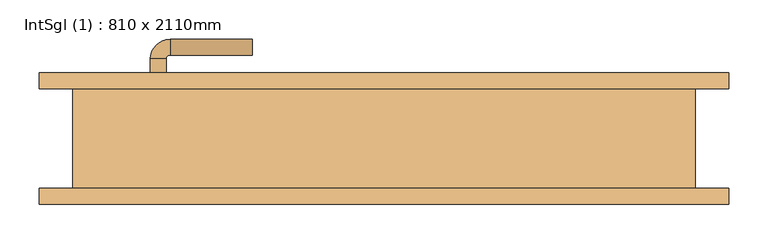
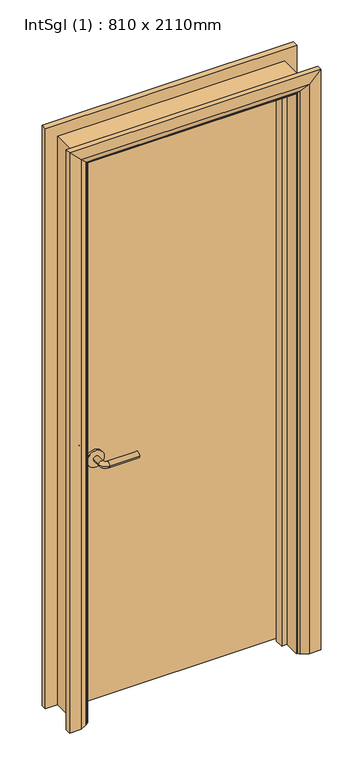
"""IFC4 building model written with IfcOpenShell, lengths in millimetres: door geometry, IntSgl (1) : 810 x 2110mm."""

from ifc_helpers import new_model, si_unit, point, frame, frame_2d, origin, place, context, project, spatial, polyline, circle_curve, ellipse_curve, trimmed, segment, composite_curve, outline, extrude, faceted_brep, source, transform, mapped, element, save
from ifc_brep_helpers import plane_surface, cylinder_surface, revolved_surface, advanced_brep


def intsgl_1_810_x_2110mm_e12ef41f(model_context):
    return source(origin(), model_context, "Body", "SolidModel", [
        advanced_brep(
        [(-298.0, 17.75, 900.0), (-278.0, 17.75, 900.0), (-278.0, -12.25, 900.0), (-298.0, -12.25, 900.0), (-273.0, -17.25, 900.0), (-273.0, -37.25, 900.0), (-168.0, -37.25, 900.0), (-168.0, -17.25, 900.0)],
        [
            (0, 1, circle_curve(frame((-288.0, 17.75, 900.0), z_axis=(0.0, 1.0, 0.0), x_axis=(1.0, 0.0, 0.0)), 10.0)),
            (1, 0, circle_curve(frame((-288.0, 17.75, 900.0), z_axis=(0.0, 1.0, 0.0), x_axis=(1.0, 0.0, 0.0)), 10.0)),
            (1, 2),
            (2, 3, circle_curve(frame((-288.0, -12.25, 900.0), z_axis=(0.0, 1.0, 0.0), x_axis=(1.0, 0.0, 0.0)), 10.0)),
            (3, 0),
            (3, 2, circle_curve(frame((-288.0, -12.25, 900.0), z_axis=(0.0, 1.0, 0.0), x_axis=(1.0, 0.0, 0.0)), 10.0)),
            (4, 5, circle_curve(frame((-273.0, -27.25, 900.0), z_axis=(-1.0, 0.0, 0.0), x_axis=(0.0, 1.0, 0.0)), 10.0)),
            (5, 3, circle_curve(frame((-273.0, -12.25, 900.0), z_axis=(0.0, 0.0, -1.0), x_axis=(-1.0, 0.0, 0.0)), 25.0)),
            (2, 4, circle_curve(frame((-273.0, -12.25, 900.0), z_axis=(0.0, 0.0, 1.0), x_axis=(-1.0, 0.0, 0.0)), 5.0)),
            (5, 4, circle_curve(frame((-273.0, -27.25, 900.0), z_axis=(-1.0, 0.0, 0.0), x_axis=(0.0, 1.0, 0.0)), 10.0)),
            (6, 7, circle_curve(frame((-168.0, -27.25, 900.0), z_axis=(1.0, 0.0, 0.0), x_axis=(0.0, 1.0, 0.0)), 10.0)),
            (7, 6, circle_curve(frame((-168.0, -27.25, 900.0), z_axis=(1.0, 0.0, 0.0), x_axis=(0.0, 1.0, 0.0)), 10.0)),
            (4, 7),
            (6, 5),
        ],
        [
            plane_surface(frame((-288.0, 17.75, 900.0), z_axis=(0.0, 1.0, 0.0), x_axis=(0.0, 0.0, 1.0))),
            cylinder_surface(frame((-288.0, 17.75, 900.0), z_axis=(0.0, 1.0, 0.0), x_axis=(1.0, 0.0, 0.0)), 10.0),
            revolved_surface(trimmed(ellipse_curve(frame((-288.0, -12.25, 900.0), z_axis=(0.0, -1.0, 0.0), x_axis=(1.0, 0.0, 0.0)), 10.0, 10.0), [point((-298.0, -12.25, 900.0))], [point((-278.0, -12.25, 900.0))], True, "CARTESIAN"), (-273.0, -12.25, 900.0), (0.0, 0.0, -1.0)),
            revolved_surface(trimmed(ellipse_curve(frame((-288.0, -12.25, 900.0), z_axis=(0.0, -1.0, 0.0), x_axis=(1.0, 0.0, 0.0)), 10.0, 10.0), [point((-278.0, -12.25, 900.0))], [point((-298.0, -12.25, 900.0))], True, "CARTESIAN"), (-273.0, -12.25, 900.0), (0.0, 0.0, -1.0)),
            plane_surface(frame((-168.0, -27.25, 900.0), z_axis=(1.0, 0.0, 0.0), x_axis=(0.0, 0.0, 1.0))),
            cylinder_surface(frame((-273.0, -27.25, 900.0), z_axis=(-1.0, 0.0, 0.0), x_axis=(0.0, 1.0, 0.0)), 10.0),
        ],
        [
            (0, [[1, 2]]),
            (1, [[3, 4, 5, -2]]),
            (1, [[-5, 6, -3, -1]]),
            (2, [[7, 8, -4, 9]]),
            (3, [[10, -9, -6, -8]]),
            (4, [[11, 12]]),
            (5, [[13, -11, 14, -7]]),
            (5, [[-14, -12, -13, -10]]),
        ],
    ),
        extrude(outline(composite_curve([segment(trimmed(circle_curve(frame_2d((900.0, -290.5)), 30.0), [point((900.0, -320.5))], [point((900.0, -260.5))], False, "CARTESIAN"), True, "CONTINUOUS"), segment(trimmed(circle_curve(frame_2d((900.0, -290.5)), 30.0), [point((900.0, -260.5))], [point((900.0, -320.5))], False, "CARTESIAN"), True, "CONTINUOUS")], self_intersect=False)), frame((0.0, 17.75, 0.0), z_axis=(0.0, 1.0, 0.0), x_axis=(0.0, 0.0, 1.0)), (0.0, 0.0, 1.0), 8.0),
        advanced_brep(
        [(-298.0, 71.75, 900.0), (-278.0, 71.75, 900.0), (-298.0, 101.75, 900.0), (-278.0, 101.75, 900.0), (-273.0, 106.75, 900.0), (-273.0, 126.75, 900.0), (-168.0, 126.75, 900.0), (-168.0, 106.75, 900.0)],
        [
            (0, 1, circle_curve(frame((-288.0, 71.75, 900.0), z_axis=(0.0, -1.0, 0.0), x_axis=(1.0, 0.0, 0.0)), 10.0)),
            (1, 0, circle_curve(frame((-288.0, 71.75, 900.0), z_axis=(0.0, -1.0, 0.0), x_axis=(1.0, 0.0, 0.0)), 10.0)),
            (0, 2),
            (2, 3, circle_curve(frame((-288.0, 101.75, 900.0), z_axis=(0.0, -1.0, 0.0), x_axis=(1.0, 0.0, 0.0)), 10.0)),
            (3, 1),
            (3, 2, circle_curve(frame((-288.0, 101.75, 900.0), z_axis=(0.0, -1.0, 0.0), x_axis=(1.0, 0.0, 0.0)), 10.0)),
            (4, 3, circle_curve(frame((-273.0, 101.75, 900.0), z_axis=(0.0, 0.0, 1.0), x_axis=(-1.0, 0.0, 0.0)), 5.0)),
            (2, 5, circle_curve(frame((-273.0, 101.75, 900.0), z_axis=(0.0, 0.0, -1.0), x_axis=(-1.0, 0.0, 0.0)), 25.0)),
            (5, 4, circle_curve(frame((-273.0, 116.75, 900.0), z_axis=(-1.0, 0.0, 0.0), x_axis=(0.0, -1.0, 0.0)), 10.0)),
            (4, 5, circle_curve(frame((-273.0, 116.75, 900.0), z_axis=(-1.0, 0.0, 0.0), x_axis=(0.0, -1.0, 0.0)), 10.0)),
            (6, 7, circle_curve(frame((-168.0, 116.75, 900.0), z_axis=(1.0, 0.0, 0.0), x_axis=(0.0, -1.0, 0.0)), 10.0)),
            (7, 6, circle_curve(frame((-168.0, 116.75, 900.0), z_axis=(1.0, 0.0, 0.0), x_axis=(0.0, -1.0, 0.0)), 10.0)),
            (5, 6),
            (7, 4),
        ],
        [
            plane_surface(frame((-288.0, 71.75, 900.0), z_axis=(0.0, -1.0, 0.0), x_axis=(0.0, 0.0, 1.0))),
            cylinder_surface(frame((-288.0, 71.75, 900.0), z_axis=(0.0, -1.0, 0.0), x_axis=(1.0, 0.0, 0.0)), 10.0),
            revolved_surface(trimmed(ellipse_curve(frame((-288.0, 101.75, 900.0), z_axis=(0.0, -1.0, 0.0), x_axis=(1.0, 0.0, 0.0)), 10.0, 10.0), [point((-298.0, 101.75, 900.0))], [point((-278.0, 101.75, 900.0))], True, "CARTESIAN"), (-273.0, 101.75, 900.0), (0.0, 0.0, -1.0)),
            revolved_surface(trimmed(ellipse_curve(frame((-288.0, 101.75, 900.0), z_axis=(0.0, -1.0, 0.0), x_axis=(1.0, 0.0, 0.0)), 10.0, 10.0), [point((-278.0, 101.75, 900.0))], [point((-298.0, 101.75, 900.0))], True, "CARTESIAN"), (-273.0, 101.75, 900.0), (0.0, 0.0, -1.0)),
            plane_surface(frame((-168.0, 116.75, 900.0), z_axis=(1.0, 0.0, 0.0), x_axis=(0.0, 0.0, 1.0))),
            cylinder_surface(frame((-273.0, 116.75, 900.0), z_axis=(-1.0, 0.0, 0.0), x_axis=(0.0, -1.0, 0.0)), 10.0),
        ],
        [
            (0, [[1, 2]]),
            (1, [[-1, 3, 4, 5]]),
            (1, [[-2, -5, 6, -3]]),
            (2, [[7, -4, 8, 9]]),
            (3, [[-8, -6, -7, 10]]),
            (4, [[11, 12]]),
            (5, [[-9, 13, -12, 14]]),
            (5, [[-10, -14, -11, -13]]),
        ],
    ),
        extrude(outline(composite_curve([segment(trimmed(circle_curve(frame_2d((900.0, -290.5)), 30.0), [point((900.0, -320.5))], [point((900.0, -260.5))], False, "CARTESIAN"), True, "CONTINUOUS"), segment(trimmed(circle_curve(frame_2d((900.0, -290.5)), 30.0), [point((900.0, -260.5))], [point((900.0, -320.5))], False, "CARTESIAN"), True, "CONTINUOUS")], self_intersect=False)), frame((0.0, 63.75, 0.0), z_axis=(0.0, 1.0, 0.0), x_axis=(0.0, 0.0, 1.0)), (0.0, 0.0, 1.0), 8.0),
        extrude(outline(polyline([(363.0, 25.75), (-363.0, 25.75), (-363.0, 63.75), (363.0, 63.75), (363.0, 25.75)])), frame((0.0, 0.0, 8.0), z_axis=(0.0, 0.0, 1.0), x_axis=(1.0, 0.0, 0.0)), (0.0, 0.0, 1.0), 2060.0),
        advanced_brep(
        [(440.0, 83.75, 0.0), (440.0, 63.75, 0.0), (370.0, 63.75, 0.0), (374.0, 69.75, 0.0), (400.0, 83.75, 0.0), (440.0, 83.75, 2145.0), (440.0, 63.75, 2145.0), (-440.0, 63.75, 2145.0), (-440.0, 63.75, 0.0), (-370.0, 63.75, 0.0), (-370.0, 63.75, 2075.0), (370.0, 63.75, 2075.0), (374.0, 69.75, 2079.0), (400.0, 83.75, 2105.0), (-400.0, 83.75, 2105.0), (-400.0, 83.75, 0.0), (-440.0, 83.75, 0.0), (-440.0, 83.75, 2145.0), (-374.0, 69.75, 2079.0), (-374.0, 69.75, 0.0)],
        [
            (0, 1),
            (1, 2),
            (2, 3, circle_curve(frame((378.0, 62.75, 0.0), z_axis=(0.0, 0.0, -1.0), x_axis=(1.0, 0.0, 0.0)), 8.0622577)),
            (3, 4),
            (4, 0),
            (0, 5),
            (5, 6),
            (6, 1),
            (6, 7),
            (7, 8),
            (8, 9),
            (9, 10),
            (10, 11),
            (11, 2),
            (11, 12, ellipse_curve(frame((378.0, 62.75, 2083.0), z_axis=(0.7071067811865475, 0.0, -0.7071067811865475), x_axis=(-0.7071067811865474, 0.0, -0.7071067811865476)), 11.4017543, 8.0622577)),
            (12, 3),
            (12, 13),
            (13, 4),
            (13, 14),
            (14, 15),
            (15, 16),
            (16, 17),
            (17, 5),
            (17, 7),
            (10, 18, ellipse_curve(frame((-378.0, 62.75, 2083.0), z_axis=(0.7071067811865475, 0.0, 0.7071067811865475), x_axis=(0.7071067811865476, 0.0, -0.7071067811865474)), 11.4017543, 8.0622577)),
            (18, 12),
            (18, 14),
            (15, 19),
            (19, 9, circle_curve(frame((-378.0, 62.75, 0.0), z_axis=(0.0, 0.0, -1.0), x_axis=(-1.0, 0.0, 0.0)), 8.0622577)),
            (8, 16),
            (19, 18),
        ],
        [
            plane_surface(frame((370.0, 63.75, 0.0), z_axis=(0.0, 0.0, -1.0), x_axis=(0.0, -1.0, 0.0))),
            plane_surface(frame((440.0, 83.75, 0.0), z_axis=(1.0, 0.0, 0.0), x_axis=(0.0, 0.0, 1.0))),
            plane_surface(frame((440.0, 63.75, 0.0), z_axis=(0.0, -1.0, 0.0), x_axis=(0.0, 0.0, 1.0))),
            cylinder_surface(frame((378.0, 62.75, 0.0), z_axis=(0.0, 0.0, -1.0), x_axis=(1.0, 0.0, 0.0)), 8.0622577),
            plane_surface(frame((374.0, 69.75, 0.0), z_axis=(-0.4740998230350126, 0.880471099922178, 0.0), x_axis=(0.0, 0.0, 1.0))),
            plane_surface(frame((400.0, 83.75, 0.0), z_axis=(0.0, 1.0, 0.0), x_axis=(0.0, 0.0, 1.0))),
            plane_surface(frame((440.0, 83.75, 2145.0), z_axis=(0.0, 0.0, 1.0), x_axis=(-1.0, 0.0, 0.0))),
            cylinder_surface(frame((370.0, 62.75, 2083.0), z_axis=(1.0, 0.0, 0.0), x_axis=(0.0, 0.0, 1.0)), 8.0622577),
            plane_surface(frame((374.0, 69.75, 2079.0), z_axis=(0.0, 0.8804710999221764, -0.4740998230350154), x_axis=(-1.0, 0.0, 0.0))),
            plane_surface(frame((-370.0, 63.75, 0.0), z_axis=(0.0, 0.0, -1.0), x_axis=(0.0, -1.0, 0.0))),
            plane_surface(frame((-440.0, 83.75, 2145.0), z_axis=(-1.0, 0.0, 0.0), x_axis=(0.0, 0.0, -1.0))),
            cylinder_surface(frame((-378.0, 62.75, 2075.0), z_axis=(0.0, 0.0, 1.0), x_axis=(-1.0, 0.0, 0.0)), 8.0622577),
            plane_surface(frame((-374.0, 69.75, 2079.0), z_axis=(0.47409982303501824, 0.8804710999221749, 0.0), x_axis=(0.0, 0.0, -1.0))),
        ],
        [
            (0, [[1, 2, 3, 4, 5]]),
            (1, [[-1, 6, 7, 8]]),
            (2, [[-2, -8, 9, 10, 11, 12, 13, 14]]),
            (3, [[-3, -14, 15, 16]]),
            (4, [[-4, -16, 17, 18]]),
            (5, [[-5, -18, 19, 20, 21, 22, 23, -6]]),
            (6, [[-7, -23, 24, -9]]),
            (7, [[-15, -13, 25, 26]]),
            (8, [[-17, -26, 27, -19]]),
            (9, [[-21, 28, 29, -11, 30]]),
            (10, [[-24, -22, -30, -10]]),
            (11, [[-25, -12, -29, 31]]),
            (12, [[-27, -31, -28, -20]]),
        ],
    ),
        extrude(outline(polyline([(0.0, -365.0), (0.0, -346.0), (2051.0, -346.0), (2051.0, 346.0), (0.0, 346.0), (0.0, 365.0), (2070.0, 365.0), (2070.0, -365.0), (0.0, -365.0)])), frame((0.0, -8.25, 0.0), z_axis=(0.0, 1.0, 0.0), x_axis=(0.0, 0.0, 1.0)), (0.0, 0.0, 1.0), 32.0),
        advanced_brep(
        [(-440.0, -83.75, 0.0), (-440.0, -63.75, 0.0), (-370.0, -63.75, 0.0), (-374.0, -69.75, 0.0), (-400.0, -83.75, 0.0), (-440.0, -83.75, 2145.0), (-440.0, -63.75, 2145.0), (-370.0, -63.75, 2075.0), (-374.0, -69.75, 2079.0), (-400.0, -83.75, 2105.0), (440.0, -83.75, 2145.0), (440.0, -63.75, 2145.0), (370.0, -63.75, 2075.0), (374.0, -69.75, 2079.0), (400.0, -83.75, 2105.0), (440.0, -83.75, 0.0), (400.0, -83.75, 0.0), (374.0, -69.75, 0.0), (370.0, -63.75, 0.0), (440.0, -63.75, 0.0)],
        [
            (0, 1),
            (1, 2),
            (2, 3, circle_curve(frame((-378.0, -62.75, 0.0), z_axis=(0.0, 0.0, -1.0), x_axis=(-1.0, 0.0, 0.0)), 8.0622577)),
            (3, 4),
            (4, 0),
            (0, 5),
            (5, 6),
            (6, 1),
            (6, 7),
            (7, 2),
            (7, 8, ellipse_curve(frame((-378.0, -62.75, 2083.0), z_axis=(-0.7071067811865475, 0.0, -0.7071067811865475), x_axis=(0.7071067811865474, 0.0, -0.7071067811865476)), 11.4017543, 8.0622577)),
            (8, 3),
            (8, 9),
            (9, 4),
            (9, 5),
            (5, 10),
            (10, 11),
            (11, 6),
            (11, 12),
            (12, 7),
            (12, 13, ellipse_curve(frame((378.0, -62.75, 2083.0), z_axis=(-0.7071067811865475, 0.0, 0.7071067811865475), x_axis=(-0.7071067811865476, 0.0, -0.7071067811865474)), 11.4017543, 8.0622577)),
            (13, 8),
            (13, 14),
            (14, 9),
            (14, 10),
            (15, 16),
            (16, 17),
            (17, 18, circle_curve(frame((378.0, -62.75, 0.0), z_axis=(0.0, 0.0, -1.0), x_axis=(1.0, 0.0, 0.0)), 8.0622577)),
            (18, 19),
            (19, 15),
            (10, 15),
            (19, 11),
            (18, 12),
            (17, 13),
            (16, 14),
        ],
        [
            plane_surface(frame((-370.0, -136.5510989, 0.0), z_axis=(0.0, 0.0, -1.0), x_axis=(1.0, 0.0, 0.0))),
            plane_surface(frame((-440.0, -83.75, 0.0), z_axis=(-1.0, 0.0, 0.0), x_axis=(0.0, 0.0, 1.0))),
            plane_surface(frame((-440.0, -63.75, 0.0), z_axis=(0.0, 1.0, 0.0), x_axis=(0.0, 0.0, 1.0))),
            cylinder_surface(frame((-378.0, -62.75, 0.0), z_axis=(0.0, 0.0, -1.0), x_axis=(-1.0, 0.0, 0.0)), 8.0622577),
            plane_surface(frame((-374.0, -69.75, 0.0), z_axis=(0.4740998230350183, -0.8804710999221749, 0.0), x_axis=(0.0, 0.0, 1.0))),
            plane_surface(frame((-400.0, -83.75, 0.0), z_axis=(0.0, -1.0, 0.0), x_axis=(0.0, 0.0, 1.0))),
            plane_surface(frame((-440.0, -83.75, 2145.0), z_axis=(0.0, 0.0, 1.0), x_axis=(1.0, 0.0, 0.0))),
            plane_surface(frame((-440.0, -63.75, 2145.0), z_axis=(0.0, 1.0, 0.0), x_axis=(1.0, 0.0, 0.0))),
            cylinder_surface(frame((-370.0, -62.75, 2083.0), z_axis=(-1.0, 0.0, 0.0), x_axis=(0.0, 0.0, 1.0)), 8.0622577),
            plane_surface(frame((-374.0, -69.75, 2079.0), z_axis=(0.0, -0.8804710999221749, -0.4740998230350183), x_axis=(1.0, 0.0, 0.0))),
            plane_surface(frame((-400.0, -83.75, 2105.0), z_axis=(0.0, -1.0, 0.0), x_axis=(1.0, 0.0, 0.0))),
            plane_surface(frame((370.0, -136.5510989, 0.0), z_axis=(0.0, 0.0, -1.0), x_axis=(-1.0, 0.0, 0.0))),
            plane_surface(frame((440.0, -83.75, 2145.0), z_axis=(1.0, 0.0, 0.0), x_axis=(0.0, 0.0, -1.0))),
            plane_surface(frame((440.0, -63.75, 2145.0), z_axis=(0.0, 1.0, 0.0), x_axis=(0.0, 0.0, -1.0))),
            cylinder_surface(frame((378.0, -62.75, 2075.0), z_axis=(0.0, 0.0, 1.0), x_axis=(1.0, 0.0, 0.0)), 8.0622577),
            plane_surface(frame((374.0, -69.75, 2079.0), z_axis=(-0.4740998230350183, -0.8804710999221749, 0.0), x_axis=(0.0, 0.0, -1.0))),
            plane_surface(frame((400.0, -83.75, 2105.0), z_axis=(0.0, -1.0, 0.0), x_axis=(0.0, 0.0, -1.0))),
        ],
        [
            (0, [[1, 2, 3, 4, 5]]),
            (1, [[-1, 6, 7, 8]]),
            (2, [[-2, -8, 9, 10]]),
            (3, [[-3, -10, 11, 12]]),
            (4, [[-4, -12, 13, 14]]),
            (5, [[-5, -14, 15, -6]]),
            (6, [[-7, 16, 17, 18]]),
            (7, [[-9, -18, 19, 20]]),
            (8, [[-11, -20, 21, 22]]),
            (9, [[-13, -22, 23, 24]]),
            (10, [[-15, -24, 25, -16]]),
            (11, [[26, 27, 28, 29, 30]]),
            (12, [[-17, 31, -30, 32]]),
            (13, [[-19, -32, -29, 33]]),
            (14, [[-21, -33, -28, 34]]),
            (15, [[-23, -34, -27, 35]]),
            (16, [[-25, -35, -26, -31]]),
        ],
    ),
        faceted_brep([(-365.0, 63.75, 0.0), (-365.0, -63.75, 0.0), (-397.0, -63.75, 0.0), (-397.0, 63.75, 0.0), (-365.0, 63.75, 2070.0), (-365.0, -63.75, 2070.0), (-397.0, -63.75, 2102.0), (-397.0, 63.75, 2102.0), (365.0, 63.75, 2070.0), (365.0, -63.75, 2070.0), (397.0, -63.75, 2102.0), (397.0, 63.75, 2102.0), (365.0, 63.75, 0.0), (397.0, 63.75, 0.0), (397.0, -63.75, 0.0), (365.0, -63.75, 0.0)], [[[0, 1, 2, 3]], [[1, 0, 4, 5]], [[2, 1, 5, 6]], [[3, 2, 6, 7]], [[0, 3, 7, 4]], [[5, 4, 8, 9]], [[6, 5, 9, 10]], [[7, 6, 10, 11]], [[4, 7, 11, 8]], [[12, 13, 14, 15]], [[9, 8, 12, 15]], [[10, 9, 15, 14]], [[11, 10, 14, 13]], [[8, 11, 13, 12]]]),
    ])


if __name__ == "__main__":
    model = new_model("IFC4")
    model_context = context("Model", 3, world=origin())
    ifc_project = project(units=[si_unit("LENGTHUNIT", "METRE", prefix="MILLI")], contexts=[model_context])
    site = spatial("IfcSite", under=ifc_project)
    building = spatial("IfcBuilding", under=site)
    placement = place(None, origin())
    intsgl_1_810_x_2110mm_shape = intsgl_1_810_x_2110mm_e12ef41f(model_context)
    element("IfcDoor", 1, ObjectType="IntSgl (1) : 810 x 2110mm", at=placement, inside=building, context=model_context, shape_type="MappedRepresentation", body=[
        mapped(intsgl_1_810_x_2110mm_shape, transform((0.0, 0.0, 0.0), x_axis=(1.0, 0.0, 0.0), y_axis=(0.0, 1.0, 0.0), z_axis=(0.0, 0.0, 1.0))),
    ])
    save(model, "model.ifc")

# Revit data of these elements
# Type "IntSgl (1) : 810 x 2110mm"
#   Construction Type Id = "MDOOR"
#   Analytic Construction = "Metal"
#   Type Mark = "42"
#   Type Comments = "Internal Single"
#   Operation = "SingleSwingRight"
#   Manufacturer = "Revit"
#   Keynote = "L20"
#   Description = "Internal Single Door"
#   Visual Light Transmittance = 0
#   Solar Heat Gain Coefficient = 0
#   Heat Transfer Coefficient (U) = 3.7021 W/(m²·K)
#   UnderCut = 8 mm
#   Tolerance = 2 mm
#   Thickness = 38 mm
#   Structural Tolerance = 8 mm
#   StopDepth = 32 mm
#   Stop Thickness = 19 mm
#   Rough Width = 810 mm
#   Rough Height = 2110 mm
#   Height to Top Lock Rail = 1000 mm
#   Handle Z Distance = 900 mm
#   Handle X Distance = 75 mm
#   Frame Thickness = 32 mm
#   Door Panel Width = 726 mm
#   Door Panel Thickness = 38 mm
#   Door Panel Offset = 0 mm
#   Height = 2110 mm
#   Width = 810 mm
#   Door Panel Height = 2060 mm
#   Architrave Setback = 5 mm
#   Function = 0
#   Vis - Ironmongery = yes
#   Material Ironmongery = Door - Handle
#   Material Frame = Door - Frame/Mullion (1)
#   Material Door = Door - Panel
#   Material Architrave = Door - Architrave
#   Wall Closure = (empty or 0)
# Element 1 (IfcDoor, "IntSgl (1) : 810 x 2110mm")
#   Materials on its faces: "Door - Architrave", "Door - Handle", "Door - Frame/Mullion (1)", "Door - Panel"
# Materials
#   "Door - Handle": class "Miscellaneous", colour RGB 0 0 0, transparency 0, Keynote = "P21"
#   "Door - Frame/Mullion (1)": class "Wood", colour RGB 212 179 113, transparency 0, Keynote = "L20", Cost = 0
#   "Door - Panel": class "Wood", colour RGB 210 159 95, transparency 0, Keynote = "L20"
#   "Door - Architrave": class "Wood", colour RGB 154 90 5, transparency 0, Keynote = "P20"
